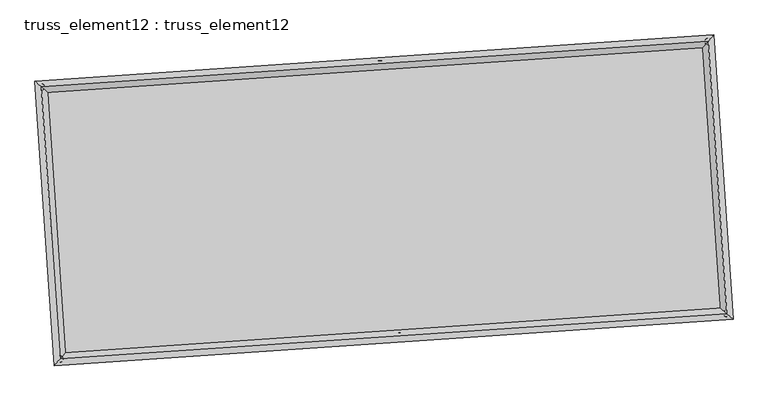
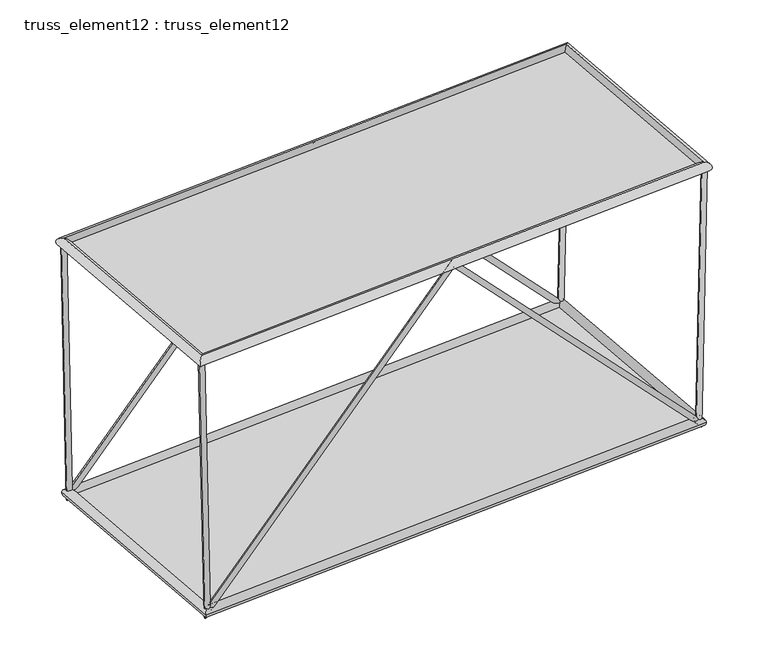
"""IFC4 building model written with IfcOpenShell, lengths in millimetres: plate geometry, truss_element12 : truss_element12."""

import ifcopenshell
import ifcopenshell.guid

model = None  # the IFC model being written
_history = None  # IfcOwnerHistory: only IFC2X3 demands one
_inside = {}  # id of a spatial element -> (the spatial element, [elements in it])
_under = {}  # id of a project, library or spatial element -> (it, [spatial elements below it])
_declared = {}  # id of a project -> (the project, [libraries it declares])
_typed = {}  # id of a type object -> (the type object, [elements of that type])
_made_of = {}  # id of a material, layer set ... -> (it, [elements and type objects made of it])


def new_model(schema):
    """Start an empty IFC model of exactly this schema.

    Asked for "IFC4X3", IfcOpenShell would pick the latest addendum, in which some entities
    have other attributes; the version numbers below select the first issue.
    IFC2X3 requires an IfcOwnerHistory on every rooted entity: one is made here for all.
    """
    global model, _history
    if schema == "IFC4X3":
        model = ifcopenshell.file(schema_version=(4, 3, 0, 0))
    else:
        model = ifcopenshell.file(schema=schema)
    _inside.clear()
    _under.clear()
    _declared.clear()
    _typed.clear()
    _made_of.clear()
    _history = None
    if model.schema == "IFC2X3":
        org = make("IfcOrganization", Name="unknown")
        user = make(
            "IfcPersonAndOrganization",
            ThePerson=make("IfcPerson", FamilyName="unknown"),
            TheOrganization=org,
        )
        app = make(
            "IfcApplication",
            ApplicationDeveloper=org,
            Version="unknown",
            ApplicationFullName="unknown",
            ApplicationIdentifier="unknown",
        )
        _history = make(
            "IfcOwnerHistory",
            OwningUser=user,
            OwningApplication=app,
            ChangeAction="ADDED",
            CreationDate=0,
        )
    return model


def make(cls, **values):
    """One entity of the class cls with the attributes given. An attribute that is None is left unset."""
    return model.create_entity(
        cls, **{name: value for name, value in values.items() if value is not None}
    )


def rooted(cls, **values):
    """An entity with a GlobalId (a new one), such as an element, a storey or a relation."""
    return make(cls, GlobalId=ifcopenshell.guid.new(), OwnerHistory=_history, **values)


def si_unit(unit_type, name, prefix=None):
    """IfcSIUnit, for example si_unit("LENGTHUNIT", "METRE", prefix="MILLI")."""
    return make("IfcSIUnit", UnitType=unit_type, Prefix=prefix, Name=name)


def assignment(units):
    """IfcUnitAssignment: the units of a project."""
    return None if units is None else make("IfcUnitAssignment", Units=units)


def point(xyz):
    """IfcCartesianPoint."""
    return None if xyz is None else make("IfcCartesianPoint", Coordinates=xyz)


def direction(xyz):
    """IfcDirection."""
    return None if xyz is None else make("IfcDirection", DirectionRatios=xyz)


def frame(location, z_axis=None, x_axis=None):
    """IfcAxis2Placement3D, a coordinate frame: its origin and axes. An axis left out is left unset."""
    return make(
        "IfcAxis2Placement3D",
        Location=point(location),
        Axis=direction(z_axis),
        RefDirection=direction(x_axis),
    )


def origin():
    """The frame at (0, 0, 0) with its axes left unset."""
    return frame((0.0, 0.0, 0.0))


def origin_with_axes():
    """The frame at (0, 0, 0) with the z axis (0, 0, 1) and the x axis (1, 0, 0) written out."""
    return frame((0.0, 0.0, 0.0), z_axis=(0.0, 0.0, 1.0), x_axis=(1.0, 0.0, 0.0))


def place(relative_to, where):
    """IfcLocalPlacement: puts the frame where relative to a parent placement (None: the world)."""
    return make(
        "IfcLocalPlacement", PlacementRelTo=relative_to, RelativePlacement=where
    )


def context(
    kind, dimensions, precision=None, world=None, true_north=None, identifier=None
):
    """IfcGeometricRepresentationContext, for example the 3D "Model" context."""
    return make(
        "IfcGeometricRepresentationContext",
        ContextIdentifier=identifier,
        ContextType=kind,
        CoordinateSpaceDimension=dimensions,
        Precision=precision,
        WorldCoordinateSystem=world,
        TrueNorth=true_north,
    )


def project(units=None, contexts=None):
    """IfcProject with its units and contexts."""
    return rooted(
        "IfcProject",
        Name="project",
        RepresentationContexts=contexts,
        UnitsInContext=assignment(units),
    )


def spatial(cls, under=None, at=None, **own):
    """A site, building, storey or space (cls), placed at a placement, below another one or the project."""
    s = rooted(cls, ObjectPlacement=at, **own)
    if under is not None:
        _under.setdefault(under.id(), (under, []))[1].append(s)
    return s


def polyline(points):
    """IfcPolyline through the points."""
    return make("IfcPolyline", Points=[point(p) for p in points])


def circle_curve(where, radius):
    """IfcCircle in the frame where."""
    return make("IfcCircle", Position=where, Radius=radius)


def ellipse_curve(where, semi_axis1, semi_axis2):
    """IfcEllipse in the frame where."""
    return make(
        "IfcEllipse", Position=where, SemiAxis1=semi_axis1, SemiAxis2=semi_axis2
    )


def outline(outer, holes=None, kind="AREA"):
    """IfcArbitraryClosedProfileDef: a profile drawn as a closed curve; with holes, ...WithVoids."""
    if holes is None:
        return make("IfcArbitraryClosedProfileDef", ProfileType=kind, OuterCurve=outer)
    return make(
        "IfcArbitraryProfileDefWithVoids",
        ProfileType=kind,
        OuterCurve=outer,
        InnerCurves=holes,
    )


def extrude(swept, where, along, depth):
    """IfcExtrudedAreaSolid: the profile swept, set in the frame where, extruded along a direction by depth."""
    return make(
        "IfcExtrudedAreaSolid",
        SweptArea=swept,
        Position=where,
        ExtrudedDirection=direction(along),
        Depth=depth,
    )


def shape(context_of_items, identifier, shape_type, items):
    """IfcShapeRepresentation: the items that make up one representation, for example the "Body"."""
    return make(
        "IfcShapeRepresentation",
        ContextOfItems=context_of_items,
        RepresentationIdentifier=identifier,
        RepresentationType=shape_type,
        Items=items,
    )


def source(mapping_origin, context_of_items, identifier, shape_type, items):
    """IfcRepresentationMap: a shape defined once, which mapped items show again and again."""
    return make(
        "IfcRepresentationMap",
        MappingOrigin=mapping_origin,
        MappedRepresentation=shape(context_of_items, identifier, shape_type, items),
    )


def transform(
    local_origin,
    x_axis=None,
    y_axis=None,
    z_axis=None,
    scale=None,
    scale2=None,
    scale3=None,
    uniform=True,
):
    """IfcCartesianTransformationOperator3D, or its non-uniform kind. x_axis, y_axis, z_axis: its Axis1, 2, 3."""
    if uniform:
        return make(
            "IfcCartesianTransformationOperator3D",
            Axis1=direction(x_axis),
            Axis2=direction(y_axis),
            LocalOrigin=point(local_origin),
            Scale=scale,
            Axis3=direction(z_axis),
        )
    return make(
        "IfcCartesianTransformationOperator3DnonUniform",
        Axis1=direction(x_axis),
        Axis2=direction(y_axis),
        LocalOrigin=point(local_origin),
        Scale=scale,
        Axis3=direction(z_axis),
        Scale2=scale2,
        Scale3=scale3,
    )


def mapped(mapping_source, mapping_target):
    """IfcMappedItem: shows the shape of a source again, moved by a transform."""
    return make(
        "IfcMappedItem", MappingSource=mapping_source, MappingTarget=mapping_target
    )


def made_of(thing, what):
    """Note that an element or type object is made of a material, layer set ...; save() writes the relation."""
    if what is not None:
        _made_of.setdefault(what.id(), (what, []))[1].append(thing)
    return thing


def element(
    cls,
    number,
    at=None,
    inside=None,
    cuts=None,
    type_object=None,
    material=None,
    context=None,
    identifier="Body",
    shape_type=None,
    held_by="IfcProductDefinitionShape",
    body=None,
    shapes=None,
    **own,
):
    """One element of the class cls, such as IfcWall. Its Tag is "e" and its number.

    at: its placement. inside: the storey or other place that contains it. cuts: it is an
    opening in that element (IfcRelVoidsElement). A single representation is given by context,
    identifier, shape_type and body (its items); several are given by shapes. held_by: the class
    of the entity that holds the representations. save() writes the other relations.
    """
    e = rooted(cls, Tag="e%d" % number, ObjectPlacement=at, **own)
    if body is not None:
        shapes = [shape(context, identifier, shape_type, body)]
    if shapes is not None:
        e.Representation = make(held_by, Representations=shapes)
    if inside is not None:
        _inside.setdefault(inside.id(), (inside, []))[1].append(e)
    if cuts is not None:
        rooted(
            "IfcRelVoidsElement", RelatingBuildingElement=cuts, RelatedOpeningElement=e
        )
    if type_object is not None:
        _typed.setdefault(type_object.id(), (type_object, []))[1].append(e)
    return made_of(e, material)


def aggregate(whole, parts):
    """IfcRelAggregates: a whole, such as a stair, and the parts it consists of."""
    return rooted("IfcRelAggregates", RelatingObject=whole, RelatedObjects=parts)


def save(model, path):
    """Write the relations noted so far, then the file.

    IfcRelAggregates (storeys below a building ...), IfcRelContainedInSpatialStructure (elements
    in a storey), IfcRelDefinesByType, IfcRelAssociatesMaterial and IfcRelDeclares: one each for
    every whole, place, type object, material and project.
    """
    for whole, parts in _under.values():
        aggregate(whole, parts)
    for where, things in _inside.values():
        rooted(
            "IfcRelContainedInSpatialStructure",
            RelatedElements=things,
            RelatingStructure=where,
        )
    for kind, things in _typed.values():
        rooted("IfcRelDefinesByType", RelatedObjects=things, RelatingType=kind)
    for what, things in _made_of.values():
        rooted("IfcRelAssociatesMaterial", RelatedObjects=things, RelatingMaterial=what)
    for by, libraries in _declared.values():
        rooted("IfcRelDeclares", RelatingContext=by, RelatedDefinitions=libraries)
    model.write(path)


def plane_surface(at):
    """IfcPlane: the flat surface through the origin of the frame at, square to its z axis."""
    return make("IfcPlane", Position=at)


def cylinder_surface(at, radius):
    """IfcCylindricalSurface: all points at the distance radius from the z axis of the frame at."""
    return make("IfcCylindricalSurface", Position=at, Radius=radius)


def advanced_brep(points, edges, surfaces, faces):
    """IfcAdvancedBrep: a solid bounded by faces that lie on surfaces and meet in shared edges.

    An edge is (start, end): straight between two places in points (the first is 0);
    or (start, end, curve); or (start, end, curve, False) where it runs against its curve.
    A face is (place in surfaces, loops), or (place, loops, False) where it looks against
    its surface's normal. A loop lists edges by number (the first is 1), with a minus sign
    where the edge is run from its end to its start. The first loop is the outer one.
    """
    corners = [point(p) for p in points]
    vertices = [make("IfcVertexPoint", VertexGeometry=c) for c in corners]
    made = []
    for start, end, *more in edges:
        made.append(
            make(
                "IfcEdgeCurve",
                EdgeStart=vertices[start],
                EdgeEnd=vertices[end],
                EdgeGeometry=more[0] if more else make("IfcPolyline", Points=[corners[start], corners[end]]),
                SameSense=more[1] if len(more) > 1 else True,
            )
        )
    hull = []
    for where, loops, *sense in faces:
        bounds = []
        for j, loop in enumerate(loops):
            ring = [make("IfcOrientedEdge", EdgeElement=made[abs(k) - 1], Orientation=k > 0) for k in loop]
            bounds.append(
                make(
                    "IfcFaceOuterBound" if j == 0 else "IfcFaceBound",
                    Bound=make("IfcEdgeLoop", EdgeList=ring),
                    Orientation=True,
                )
            )
        hull.append(make("IfcAdvancedFace", Bounds=bounds, FaceSurface=surfaces[where], SameSense=sense[0] if sense else True))
    return make("IfcAdvancedBrep", Outer=make("IfcClosedShell", CfsFaces=hull))


def truss_element12_truss_element12_086eec47(model_context):
    return source(origin(), model_context, "Body", "SolidModel", [
        advanced_brep(
        [(-3774.2332872, 2268.7717745, 4999.8930544), (-3873.3127666, 2255.4121866, 4997.7071475), (-3667.5840303, 2276.0437819, 121.4126505), (-3761.4028525, 2263.0428982, -121.4126505), (1064.2299582, 2598.6881905, 5070.9037686), (1064.6705353, 2592.1144969, 4926.674072), (5795.0471287, 2921.2646298, 121.4057099), (5889.7138483, 2921.1158587, -121.4057099), (5902.6858035, 2928.6041019, 4999.8808289), (6002.6612371, 2928.8173118, 4997.6746502)],
        [
            (0, 1, circle_curve(frame((-3823.7730269, 2262.0919805, 4998.800101), z_axis=(-0.021855917096439963, -0.0014902719046873062, 0.9997600201936082), x_axis=(-0.13359639491826203, 0.9910347724122863, -0.0014433068183134015)), 50.0)),
            (1, 0, circle_curve(frame((-3823.7730269, 2262.0919805, 4998.800101), z_axis=(-0.021855917096439963, -0.0014902719046873062, 0.9997600201936082), x_axis=(-0.13359639491826203, 0.9910347724122863, -0.0014433068183134015)), 50.0)),
            (0, 2),
            (2, 3, ellipse_curve(frame((-3714.4934414, 2269.54334, 0.0), z_axis=(-0.9297759208968324, -0.06339788563679134, 0.3626257644145429), x_axis=(0.3617857041453493, 0.024668791889457715, 0.9319348448162931)), 130.5638727, 50.0)),
            (3, 1),
            (3, 2, ellipse_curve(frame((-3714.4934414, 2269.54334, 0.0), z_axis=(-0.9297759208968324, -0.06339788563679134, 0.3626257644145429), x_axis=(0.3617857041453493, 0.024668791889457715, 0.9319348448162931)), 130.5638727, 50.0)),
            (2, 4),
            (4, 5, ellipse_curve(frame((1064.4502467, 2595.4013437, 4998.7889203), z_axis=(-0.9976833946750359, -0.06802823813325232, 5.297341116267986e-05), x_axis=(-5.285069275020394e-05, -3.6036878343152564e-06, -0.9999999985969089)), 72.2718761, 50.0)),
            (5, 3),
            (5, 4, ellipse_curve(frame((1064.4502467, 2595.4013437, 4998.7889203), z_axis=(-0.9976833946750359, -0.06802823813325232, 5.297341116267986e-05), x_axis=(-5.285069275020394e-05, -3.6036878343152564e-06, -0.9999999985969089)), 72.2718761, 50.0)),
            (4, 6),
            (6, 7, ellipse_curve(frame((5842.3804885, 2921.1902443, 0.0), z_axis=(-0.9298318338903021, -0.06340169813127101, -0.36248170348069864), x_axis=(-0.3616419769436296, -0.024658991677930685, 0.9319908876387853)), 130.5485583, 50.0)),
            (7, 5),
            (7, 6, ellipse_curve(frame((5842.3804885, 2921.1902443, 0.0), z_axis=(-0.9298318338903021, -0.06340169813127101, -0.36248170348069864), x_axis=(-0.3616419769436296, -0.024658991677930685, 0.9319908876387853)), 130.5485583, 50.0)),
            (8, 9, circle_curve(frame((5952.6735203, 2928.7107068, 4998.7777396), z_axis=(0.022058606365204667, 0.0015040925154303942, 0.9997555479170547), x_axis=(-0.002164760807071468, 0.9999965959239133, -0.00145669188023135)), 50.0)),
            (9, 8, circle_curve(frame((5952.6735203, 2928.7107068, 4998.7777396), z_axis=(0.022058606365204667, 0.0015040925154303942, 0.9997555479170547), x_axis=(-0.002164760807071468, 0.9999965959239133, -0.00145669188023135)), 50.0)),
            (6, 8),
            (9, 7),
        ],
        [
            plane_surface(frame((-3823.7730269, 2312.091925, 4998.8746324), z_axis=(-0.021855917096441312, -0.0014902719046848139, 0.9997600201936081), x_axis=(0.9997611309147169, -3.257904132603074e-05, 0.02185589281481271))),
            cylinder_surface(frame((-3823.7730269, 2262.0919805, 4998.800101), z_axis=(-0.021855917096439963, -0.0014902719046873062, 0.9997600201936082), x_axis=(-0.13359639491826203, 0.9910347724122863, -0.0014433068183134015)), 50.0),
            cylinder_surface(frame((-3714.4934414, 2269.54334, 0.0), z_axis=(-0.6902675071609972, -0.0470667173608615, -0.7220218090020663), x_axis=(-0.020420682259035285, 0.9987517940373583, -0.04558343606217084)), 50.0),
            cylinder_surface(frame((1064.4502467, 2595.4013437, 4998.7889203), z_axis=(-0.6901911845814975, -0.04706151321429475, 0.7220951064091002), x_axis=(-0.11534499746176513, 0.9922792658247876, -0.045578395921375275)), 50.0),
            plane_surface(frame((5952.6735203, 2878.7107634, 4998.8529625), z_axis=(0.022058606365203737, 0.0015040925154315723, 0.9997555479170548), x_axis=(0.9997566793401409, -3.318625963721899e-05, -0.022058581401513063))),
            cylinder_surface(frame((5842.3804885, 2921.1902443, 0.0), z_axis=(-0.022058606365204667, -0.0015040925154303942, -0.9997555479170547), x_axis=(-0.002164760807071468, 0.9999965959239133, -0.00145669188023135)), 50.0),
        ],
        [
            (0, [[1, 2]]),
            (1, [[-1, 3, 4, 5]]),
            (1, [[-2, -5, 6, -3]]),
            (2, [[-4, 7, 8, 9]]),
            (2, [[-6, -9, 10, -7]]),
            (3, [[-8, 11, 12, 13]]),
            (3, [[-10, -13, 14, -11]]),
            (4, [[15, 16]]),
            (5, [[-12, 17, -16, 18]]),
            (5, [[-14, -18, -15, -17]]),
        ],
    ),
        advanced_brep(
        [(-3502.1203343, -1721.9618098, 4999.8930544), (-3601.1998136, -1735.3213977, 4997.7071475), (-3395.4710774, -1714.6898024, 121.4126505), (-3489.2898996, -1727.6906861, -121.4126505), (1336.3429111, -1392.0453938, 5070.9037686), (1336.7834882, -1398.6190874, 4926.674072), (6067.1600816, -1069.4689545, 121.4057099), (6161.8268012, -1069.6177256, -121.4057099), (6174.7987565, -1062.1294824, 4999.8808289), (6274.77419, -1061.9162725, 4997.6746502)],
        [
            (0, 1, circle_curve(frame((-3551.660074, -1728.6416038, 4998.800101), z_axis=(-0.02185591709644024, -0.001490271904687352, 0.9997600201936082), x_axis=(-0.13359639491826175, 0.9910347724122863, -0.0014433068183133876)), 50.0)),
            (1, 0, circle_curve(frame((-3551.660074, -1728.6416038, 4998.800101), z_axis=(-0.02185591709644024, -0.001490271904687352, 0.9997600201936082), x_axis=(-0.13359639491826175, 0.9910347724122863, -0.0014433068183133876)), 50.0)),
            (0, 2),
            (2, 3, ellipse_curve(frame((-3442.3804885, -1721.1902443, 0.0), z_axis=(-0.9297759208968323, -0.06339788563679132, 0.36262576441454303), x_axis=(0.3617857041453494, 0.024668791889457687, 0.9319348448162932)), 130.5638727, 50.0)),
            (3, 1),
            (3, 2, ellipse_curve(frame((-3442.3804885, -1721.1902443, 0.0), z_axis=(-0.9297759208968323, -0.06339788563679132, 0.36262576441454303), x_axis=(0.3617857041453494, 0.024668791889457687, 0.9319348448162932)), 130.5638727, 50.0)),
            (2, 4),
            (4, 5, ellipse_curve(frame((1336.5631996, -1395.3322406, 4998.7889203), z_axis=(-0.9976833946750359, -0.06802823813325233, 5.2973411162840336e-05), x_axis=(-5.285069275035771e-05, -3.6036878342575984e-06, -0.9999999985969089)), 72.2718761, 50.0)),
            (5, 3),
            (5, 4, ellipse_curve(frame((1336.5631996, -1395.3322406, 4998.7889203), z_axis=(-0.9976833946750359, -0.06802823813325233, 5.2973411162840336e-05), x_axis=(-5.285069275035771e-05, -3.6036878342575984e-06, -0.9999999985969089)), 72.2718761, 50.0)),
            (4, 6),
            (6, 7, ellipse_curve(frame((6114.4934414, -1069.54334, 0.0), z_axis=(-0.9298318338903019, -0.06340169813127097, -0.3624817034806985), x_axis=(-0.3616419769436298, -0.024658991677930772, 0.9319908876387852)), 130.5485583, 50.0)),
            (7, 5),
            (7, 6, ellipse_curve(frame((6114.4934414, -1069.54334, 0.0), z_axis=(-0.9298318338903019, -0.06340169813127097, -0.3624817034806985), x_axis=(-0.3616419769436298, -0.024658991677930772, 0.9319908876387852)), 130.5485583, 50.0)),
            (8, 9, circle_curve(frame((6224.7864732, -1062.0228775, 4998.7777396), z_axis=(0.022058606365204722, 0.0015040925154303226, 0.9997555479170547), x_axis=(-0.0021647608070713776, 0.9999965959239133, -0.0014566918802312804)), 50.0)),
            (9, 8, circle_curve(frame((6224.7864732, -1062.0228775, 4998.7777396), z_axis=(0.022058606365204722, 0.0015040925154303226, 0.9997555479170547), x_axis=(-0.0021647608070713776, 0.9999965959239133, -0.0014566918802312804)), 50.0)),
            (6, 8),
            (9, 7),
        ],
        [
            plane_surface(frame((-3551.660074, -1678.6416593, 4998.8746324), z_axis=(-0.021855917096441312, -0.0014902719046848097, 0.9997600201936081), x_axis=(0.9997611309147169, -3.257904132603074e-05, 0.02185589281481271))),
            cylinder_surface(frame((-3551.660074, -1728.6416038, 4998.800101), z_axis=(-0.02185591709644024, -0.001490271904687352, 0.9997600201936082), x_axis=(-0.13359639491826175, 0.9910347724122863, -0.0014433068183133876)), 50.0),
            cylinder_surface(frame((-3442.3804885, -1721.1902443, 0.0), z_axis=(-0.6902675071609972, -0.04706671736086146, -0.722021809002066), x_axis=(-0.02042068225903536, 0.9987517940373583, -0.04558343606217072)), 50.0),
            cylinder_surface(frame((1336.5631996, -1395.3322406, 4998.7889203), z_axis=(-0.6901911845814976, -0.04706151321429482, 0.7220951064091004), x_axis=(-0.11534499746176505, 0.9922792658247878, -0.04557839592137508)), 50.0),
            plane_surface(frame((6224.7864732, -1112.0228209, 4998.8529625), z_axis=(0.022058606365203737, 0.0015040925154315703, 0.9997555479170548), x_axis=(0.9997566793401409, -3.318625963721899e-05, -0.022058581401513063))),
            cylinder_surface(frame((6114.4934414, -1069.54334, 0.0), z_axis=(-0.022058606365204722, -0.0015040925154303226, -0.9997555479170547), x_axis=(-0.0021647608070713776, 0.9999965959239133, -0.0014566918802312804)), 50.0),
        ],
        [
            (0, [[1, 2]]),
            (1, [[-1, 3, 4, 5]]),
            (1, [[-2, -5, 6, -3]]),
            (2, [[-4, 7, 8, 9]]),
            (2, [[-6, -9, 10, -7]]),
            (3, [[-8, 11, 12, 13]]),
            (3, [[-10, -13, 14, -11]]),
            (4, [[15, 16]]),
            (5, [[-12, 17, -16, 18]]),
            (5, [[-14, -18, -15, -17]]),
        ],
    ),
        advanced_brep(
        [(-3551.6658856, -1728.6480451, 4908.8001012), (-3551.6542623, -1728.6351625, 5088.8001008), (-3823.7663947, 2262.0863877, 5088.8001008), (-3823.7796591, 2262.0975733, 4908.8001012), (5952.6681185, 2928.7042935, 5088.7777394), (5952.6789222, 2928.7171202, 4908.7777398), (6224.7802508, -1062.0172567, 5088.7777394), (6224.7926957, -1062.0284982, 4908.7777398)],
        [
            (0, 1, ellipse_curve(frame((-3551.660074, -1728.6416038, 4998.800101), z_axis=(-0.7535719234036229, 0.6573654662782041, 1.6135980928572344e-06), x_axis=(-0.6573654662762421, -0.7535719234053343, 1.6135980928572024e-06)), 127.2792206, 90.0)),
            (1, 2),
            (2, 3, ellipse_curve(frame((-3823.7730269, 2262.0919805, 4998.800101), z_axis=(-0.6573654662762419, -0.7535719234053345, 1.61359809285717e-06), x_axis=(0.7535719234036229, -0.6573654662782039, -1.6135980928572026e-06)), 127.2792206, 90.0)),
            (3, 0),
            (1, 0, ellipse_curve(frame((-3551.660074, -1728.6416038, 4998.800101), z_axis=(-0.7535719234036229, 0.6573654662782041, 1.6135980928572344e-06), x_axis=(-0.6573654662762421, -0.7535719234053343, 1.6135980928572024e-06)), 127.2792206, 90.0)),
            (3, 2, ellipse_curve(frame((-3823.7730269, 2262.0919805, 4998.800101), z_axis=(-0.6573654662762419, -0.7535719234053345, 1.61359809285717e-06), x_axis=(0.7535719234036229, -0.6573654662782039, -1.6135980928572026e-06)), 127.2792206, 90.0)),
            (2, 4),
            (4, 5, ellipse_curve(frame((5952.6735203, 2928.7107068, 4998.7777396), z_axis=(-0.7535719234036229, 0.657365466278204, 1.6135980928571717e-06), x_axis=(-0.657365466276242, -0.7535719234053344, 1.6135980928572015e-06)), 127.2792206, 90.0)),
            (5, 3),
            (5, 4, ellipse_curve(frame((5952.6735203, 2928.7107068, 4998.7777396), z_axis=(-0.7535719234036229, 0.657365466278204, 1.6135980928571717e-06), x_axis=(-0.657365466276242, -0.7535719234053344, 1.6135980928572015e-06)), 127.2792206, 90.0)),
            (4, 6),
            (6, 7, ellipse_curve(frame((6224.7864732, -1062.0228775, 4998.7777396), z_axis=(0.657365466276242, 0.7535719234053344, -1.6135980928572333e-06), x_axis=(-0.7535719234036229, 0.6573654662782041, 1.6135980928572032e-06)), 127.2792206, 90.0)),
            (7, 5),
            (7, 6, ellipse_curve(frame((6224.7864732, -1062.0228775, 4998.7777396), z_axis=(0.657365466276242, 0.7535719234053344, -1.6135980928572333e-06), x_axis=(-0.7535719234036229, 0.6573654662782041, 1.6135980928572032e-06)), 127.2792206, 90.0)),
            (6, 1),
            (0, 7),
        ],
        [
            cylinder_surface(frame((-3551.660074, -1728.6416038, 4998.800101), z_axis=(0.06802823822870424, -0.9976833960748764, 0.0), x_axis=(-0.9976833936796619, -0.06802823806538366, 6.929323559275387e-05)), 90.0),
            cylinder_surface(frame((-3823.7730269, 2262.0919805, 4998.800101), z_axis=(-0.997683396072279, -0.06802823822852651, 2.2819723071379943e-06), x_axis=(-0.0680282379233993, 0.997683393845226, 6.701126329073946e-05)), 90.0),
            cylinder_surface(frame((5952.6735203, 2928.7107068, 4998.7777396), z_axis=(-0.06802823822870425, 0.9976833960748764, 0.0), x_axis=(0.997683393984789, 0.06802823808618913, 6.472929098872504e-05)), 90.0),
            cylinder_surface(frame((6224.7864732, -1062.0228775, 4998.7777396), z_axis=(0.9976833960722788, 0.06802823822852633, -2.2819723071380388e-06), x_axis=(0.06802823822852633, -0.9976833938244204, 6.701126329073944e-05)), 90.0),
        ],
        [
            (0, [[1, 2, 3, 4]]),
            (0, [[5, -4, 6, -2]]),
            (1, [[-3, 7, 8, 9]]),
            (1, [[-6, -9, 10, -7]]),
            (2, [[-8, 11, 12, 13]]),
            (2, [[-10, -13, 14, -11]]),
            (3, [[-12, 15, -1, 16]]),
            (3, [[-14, -16, -5, -15]]),
        ],
    ),
        advanced_brep(
        [(-3358.7115243, -1625.2761972, 0.0), (-3526.0494527, -1817.1042913, 0.0), (-3810.4074885, 2353.2123043, 0.0), (-3618.5793943, 2185.8743758, 0.0), (5926.0494527, 3017.1042913, 0.0), (5758.7115243, 2825.2761972, 0.0), (6210.4074885, -1153.2123043, 0.0), (6018.5793943, -985.8743758, 0.0)],
        [
            (0, 1, ellipse_curve(frame((-3442.3804885, -1721.1902443, 0.0), z_axis=(-0.7535719234054589, 0.6573654662780798, 0.0), x_axis=(-0.6573654662780798, -0.7535719234054589, 0.0)), 127.2792206, 90.0)),
            (1, 2),
            (2, 3, ellipse_curve(frame((-3714.4934414, 2269.54334, 0.0), z_axis=(-0.6573654662780798, -0.7535719234054589, 0.0), x_axis=(0.7535719234054589, -0.6573654662780799, 0.0)), 127.2792206, 90.0)),
            (3, 0),
            (1, 0, ellipse_curve(frame((-3442.3804885, -1721.1902443, 0.0), z_axis=(-0.7535719234054589, 0.6573654662780798, 0.0), x_axis=(-0.6573654662780798, -0.7535719234054589, 0.0)), 127.2792206, 90.0)),
            (3, 2, ellipse_curve(frame((-3714.4934414, 2269.54334, 0.0), z_axis=(-0.6573654662780798, -0.7535719234054589, 0.0), x_axis=(0.7535719234054589, -0.6573654662780799, 0.0)), 127.2792206, 90.0)),
            (2, 4),
            (4, 5, ellipse_curve(frame((5842.3804885, 2921.1902443, 0.0), z_axis=(-0.7535719234054589, 0.6573654662780798, 0.0), x_axis=(-0.6573654662780797, -0.753571923405459, 0.0)), 127.2792206, 90.0)),
            (5, 3),
            (5, 4, ellipse_curve(frame((5842.3804885, 2921.1902443, 0.0), z_axis=(-0.7535719234054589, 0.6573654662780798, 0.0), x_axis=(-0.6573654662780797, -0.753571923405459, 0.0)), 127.2792206, 90.0)),
            (4, 6),
            (6, 7, ellipse_curve(frame((6114.4934414, -1069.54334, 0.0), z_axis=(0.6573654662780798, 0.7535719234054589, 0.0), x_axis=(-0.753571923405459, 0.6573654662780797, 0.0)), 127.2792206, 90.0)),
            (7, 5),
            (7, 6, ellipse_curve(frame((6114.4934414, -1069.54334, 0.0), z_axis=(0.6573654662780798, 0.7535719234054589, 0.0), x_axis=(-0.753571923405459, 0.6573654662780797, 0.0)), 127.2792206, 90.0)),
            (6, 1),
            (0, 7),
        ],
        [
            cylinder_surface(frame((-3442.3804885, -1721.1902443, 0.0), z_axis=(0.06802823822870296, -0.9976833960748764, 0.0), x_axis=(-0.9976833960748764, -0.06802823822870296, 0.0)), 90.0),
            cylinder_surface(frame((-3714.4934414, 2269.54334, 0.0), z_axis=(-0.9976833960748765, -0.06802823822870219, 0.0), x_axis=(-0.06802823822870219, 0.9976833960748765, 0.0)), 90.0),
            cylinder_surface(frame((5842.3804885, 2921.1902443, 0.0), z_axis=(-0.06802823822870291, 0.9976833960748764, 0.0), x_axis=(0.9976833960748764, 0.06802823822870291, 0.0)), 90.0),
            cylinder_surface(frame((6114.4934414, -1069.54334, 0.0), z_axis=(0.9976833960748765, 0.06802823822870213, 0.0), x_axis=(0.06802823822870213, -0.9976833960748765, 0.0)), 90.0),
        ],
        [
            (0, [[1, 2, 3, 4]]),
            (0, [[5, -4, 6, -2]]),
            (1, [[-3, 7, 8, 9]]),
            (1, [[-6, -9, 10, -7]]),
            (2, [[-8, 11, 12, 13]]),
            (2, [[-10, -13, 14, -11]]),
            (3, [[-12, 15, -1, 16]]),
            (3, [[-14, -16, -5, -15]]),
        ],
    ),
        extrude(outline(polyline([(-3442.3804885, -1721.1902443), (-3714.4934414, 2269.54334), (5842.3804885, 2921.1902443), (6114.4934414, -1069.54334), (-3442.3804885, -1721.1902443)])), origin_with_axes(), (0.0, 0.0, 1.0), 20.0),
        extrude(outline(polyline([(-2000.0, 4899.5736452), (2000.0, 4899.5736452), (2000.0, -4899.5736451), (-2000.0, -4899.5736451), (-2000.0, 4899.5736452)])), frame((1200.5067232, 600.0345515, 4998.7889203), z_axis=(2.2766858811342764e-06, 1.5523855574128772e-07, 0.9999999999973964), x_axis=(-0.06802823822870292, 0.9976833960748765, 0.0)), (0.0, 0.0, 1.0), 20.0),
    ])


if __name__ == "__main__":
    model = new_model("IFC4")
    model_context = context("Model", 3, world=origin())
    ifc_project = project(units=[si_unit("LENGTHUNIT", "METRE", prefix="MILLI")], contexts=[model_context])
    site = spatial("IfcSite", under=ifc_project)
    building = spatial("IfcBuilding", under=site)
    placement = place(None, origin())
    truss_element12_truss_element12_shape = truss_element12_truss_element12_086eec47(model_context)
    element("IfcPlate", 1, ObjectType="truss_element12 : truss_element12", at=placement, inside=building, context=model_context, shape_type="MappedRepresentation", body=[
        mapped(truss_element12_truss_element12_shape, transform((0.0, 0.0, 0.0), x_axis=(1.0, 0.0, 0.0), y_axis=(0.0, 1.0, 0.0), z_axis=(0.0, 0.0, 1.0))),
    ])
    save(model, "model.ifc")

# Revit data of these elements
# Project information
#   Project Issue Date = "Issue Date"
#   Project Status = "Project Status"
#   Client Name = "Owner"
#   Project Address = "Enter address here"
#   Project Name = "Project Name"
#   Project Number = "Project Number"
# Type "truss_element12 : truss_element12"
#   steellbar1 = 90 mm
#   steelbar2 = 50 mm
#   offset1 = 5000 mm
#   M = Default Roof
# Element 1 (IfcPlate, "truss_element12 : truss_element12")
#   Materials on its faces: "Default Roof"
# Materials
#   "Default Roof": class "Miscellaneous", colour RGB 0 127 0, transparency 0, Comments = "Rendering appearance not upgraded Rendering appearance not upgraded ", Cost = 0
